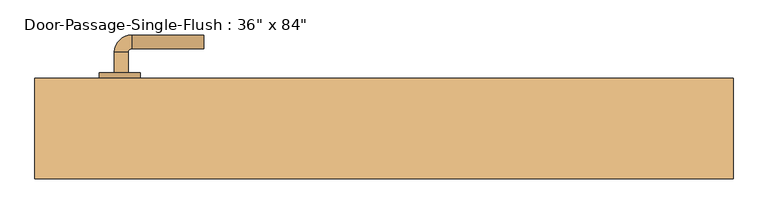
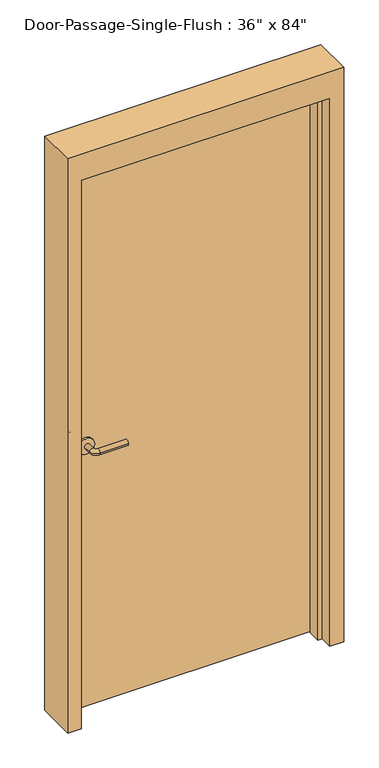
"""IFC4 building model written with IfcOpenShell, lengths in millimetres: door geometry."""

from ifc_helpers import new_model, si_unit, point, frame, frame_2d, origin, origin_with_axes, place, context, project, spatial, polyline, circle_curve, ellipse_curve, trimmed, segment, composite_curve, outline, extrude, faceted_brep, source, transform, mapped, element, save
from ifc_brep_helpers import plane_surface, cylinder_surface, revolved_surface, advanced_brep


def door_a46f4f49(model_context):
    return source(origin(), model_context, "Body", "SolidModel", [
        advanced_brep(
        [(-392.190625, 23.75, 1016.0), (-372.190625, 23.75, 1016.0), (-372.190625, -6.25, 1016.0), (-392.190625, -6.25, 1016.0), (-367.190625, -11.25, 1016.0), (-367.190625, -31.25, 1016.0), (-262.190625, -31.25, 1016.0), (-262.190625, -11.25, 1016.0)],
        [
            (0, 1, circle_curve(frame((-382.190625, 23.75, 1016.0), z_axis=(0.0, 1.0, 0.0), x_axis=(1.0, 0.0, 0.0)), 10.0)),
            (1, 0, circle_curve(frame((-382.190625, 23.75, 1016.0), z_axis=(0.0, 1.0, 0.0), x_axis=(1.0, 0.0, 0.0)), 10.0)),
            (1, 2),
            (2, 3, circle_curve(frame((-382.190625, -6.25, 1016.0), z_axis=(0.0, 1.0, 0.0), x_axis=(1.0, 0.0, 0.0)), 10.0)),
            (3, 0),
            (3, 2, circle_curve(frame((-382.190625, -6.25, 1016.0), z_axis=(0.0, 1.0, 0.0), x_axis=(1.0, 0.0, 0.0)), 10.0)),
            (4, 5, circle_curve(frame((-367.190625, -21.25, 1016.0), z_axis=(-1.0, 0.0, 0.0), x_axis=(0.0, 1.0, 0.0)), 10.0)),
            (5, 3, circle_curve(frame((-367.190625, -6.25, 1016.0), z_axis=(0.0, 0.0, -1.0), x_axis=(-1.0, 0.0, 0.0)), 25.0)),
            (2, 4, circle_curve(frame((-367.190625, -6.25, 1016.0), z_axis=(0.0, 0.0, 1.0), x_axis=(-1.0, 0.0, 0.0)), 5.0)),
            (5, 4, circle_curve(frame((-367.190625, -21.25, 1016.0), z_axis=(-1.0, 0.0, 0.0), x_axis=(0.0, 1.0, 0.0)), 10.0)),
            (6, 7, circle_curve(frame((-262.190625, -21.25, 1016.0), z_axis=(1.0, 0.0, 0.0), x_axis=(0.0, 1.0, 0.0)), 10.0)),
            (7, 6, circle_curve(frame((-262.190625, -21.25, 1016.0), z_axis=(1.0, 0.0, 0.0), x_axis=(0.0, 1.0, 0.0)), 10.0)),
            (4, 7),
            (6, 5),
        ],
        [
            plane_surface(frame((-382.190625, 23.75, 1016.0), z_axis=(0.0, 1.0, 0.0), x_axis=(0.0, 0.0, 1.0))),
            cylinder_surface(frame((-382.190625, 23.75, 1016.0), z_axis=(0.0, 1.0, 0.0), x_axis=(1.0, 0.0, 0.0)), 10.0),
            revolved_surface(trimmed(ellipse_curve(frame((-382.190625, -6.25, 1016.0), z_axis=(0.0, -1.0, 0.0), x_axis=(1.0, 0.0, 0.0)), 10.0, 10.0), [point((-392.190625, -6.25, 1016.0))], [point((-372.190625, -6.25, 1016.0))], True, "CARTESIAN"), (-367.190625, -6.25, 1016.0), (0.0, 0.0, -1.0)),
            revolved_surface(trimmed(ellipse_curve(frame((-382.190625, -6.25, 1016.0), z_axis=(0.0, -1.0, 0.0), x_axis=(1.0, 0.0, 0.0)), 10.0, 10.0), [point((-372.190625, -6.25, 1016.0))], [point((-392.190625, -6.25, 1016.0))], True, "CARTESIAN"), (-367.190625, -6.25, 1016.0), (0.0, 0.0, -1.0)),
            plane_surface(frame((-262.190625, -21.25, 1016.0), z_axis=(1.0, 0.0, 0.0), x_axis=(0.0, 0.0, 1.0))),
            cylinder_surface(frame((-367.190625, -21.25, 1016.0), z_axis=(-1.0, 0.0, 0.0), x_axis=(0.0, 1.0, 0.0)), 10.0),
        ],
        [
            (0, [[1, 2]]),
            (1, [[3, 4, 5, -2]]),
            (1, [[-5, 6, -3, -1]]),
            (2, [[7, 8, -4, 9]]),
            (3, [[10, -9, -6, -8]]),
            (4, [[11, 12]]),
            (5, [[13, -11, 14, -7]]),
            (5, [[-14, -12, -13, -10]]),
        ],
    ),
        extrude(outline(composite_curve([segment(trimmed(circle_curve(frame_2d((1016.0, -384.690625)), 30.0), [point((1016.0, -414.690625))], [point((1016.0, -354.690625))], False, "CARTESIAN"), True, "CONTINUOUS"), segment(trimmed(circle_curve(frame_2d((1016.0, -384.690625)), 30.0), [point((1016.0, -354.690625))], [point((1016.0, -414.690625))], False, "CARTESIAN"), True, "CONTINUOUS")], self_intersect=False)), frame((0.0, 23.75, 0.0), z_axis=(0.0, 1.0, 0.0), x_axis=(0.0, 0.0, 1.0)), (0.0, 0.0, 1.0), 8.0),
        advanced_brep(
        [(-392.190625, 84.2, 1016.0), (-372.190625, 84.2, 1016.0), (-392.190625, 114.2, 1016.0), (-372.190625, 114.2, 1016.0), (-367.190625, 119.2, 1016.0), (-367.190625, 139.2, 1016.0), (-262.190625, 139.2, 1016.0), (-262.190625, 119.2, 1016.0)],
        [
            (0, 1, circle_curve(frame((-382.190625, 84.2, 1016.0), z_axis=(0.0, -1.0, 0.0), x_axis=(1.0, 0.0, 0.0)), 10.0)),
            (1, 0, circle_curve(frame((-382.190625, 84.2, 1016.0), z_axis=(0.0, -1.0, 0.0), x_axis=(1.0, 0.0, 0.0)), 10.0)),
            (0, 2),
            (2, 3, circle_curve(frame((-382.190625, 114.2, 1016.0), z_axis=(0.0, -1.0, 0.0), x_axis=(1.0, 0.0, 0.0)), 10.0)),
            (3, 1),
            (3, 2, circle_curve(frame((-382.190625, 114.2, 1016.0), z_axis=(0.0, -1.0, 0.0), x_axis=(1.0, 0.0, 0.0)), 10.0)),
            (4, 3, circle_curve(frame((-367.190625, 114.2, 1016.0), z_axis=(0.0, 0.0, 1.0), x_axis=(-1.0, 0.0, 0.0)), 5.0)),
            (2, 5, circle_curve(frame((-367.190625, 114.2, 1016.0), z_axis=(0.0, 0.0, -1.0), x_axis=(-1.0, 0.0, 0.0)), 25.0)),
            (5, 4, circle_curve(frame((-367.190625, 129.2, 1016.0), z_axis=(-1.0, 0.0, 0.0), x_axis=(0.0, -1.0, 0.0)), 10.0)),
            (4, 5, circle_curve(frame((-367.190625, 129.2, 1016.0), z_axis=(-1.0, 0.0, 0.0), x_axis=(0.0, -1.0, 0.0)), 10.0)),
            (6, 7, circle_curve(frame((-262.190625, 129.2, 1016.0), z_axis=(1.0, 0.0, 0.0), x_axis=(0.0, -1.0, 0.0)), 10.0)),
            (7, 6, circle_curve(frame((-262.190625, 129.2, 1016.0), z_axis=(1.0, 0.0, 0.0), x_axis=(0.0, -1.0, 0.0)), 10.0)),
            (5, 6),
            (7, 4),
        ],
        [
            plane_surface(frame((-382.190625, 84.2, 1016.0), z_axis=(0.0, -1.0, 0.0), x_axis=(0.0, 0.0, 1.0))),
            cylinder_surface(frame((-382.190625, 84.2, 1016.0), z_axis=(0.0, -1.0, 0.0), x_axis=(1.0, 0.0, 0.0)), 10.0),
            revolved_surface(trimmed(ellipse_curve(frame((-382.190625, 114.2, 1016.0), z_axis=(0.0, -1.0, 0.0), x_axis=(1.0, 0.0, 0.0)), 10.0, 10.0), [point((-392.190625, 114.2, 1016.0))], [point((-372.190625, 114.2, 1016.0))], True, "CARTESIAN"), (-367.190625, 114.2, 1016.0), (0.0, 0.0, -1.0)),
            revolved_surface(trimmed(ellipse_curve(frame((-382.190625, 114.2, 1016.0), z_axis=(0.0, -1.0, 0.0), x_axis=(1.0, 0.0, 0.0)), 10.0, 10.0), [point((-372.190625, 114.2, 1016.0))], [point((-392.190625, 114.2, 1016.0))], True, "CARTESIAN"), (-367.190625, 114.2, 1016.0), (0.0, 0.0, -1.0)),
            plane_surface(frame((-262.190625, 129.2, 1016.0), z_axis=(1.0, 0.0, 0.0), x_axis=(0.0, 0.0, 1.0))),
            cylinder_surface(frame((-367.190625, 129.2, 1016.0), z_axis=(-1.0, 0.0, 0.0), x_axis=(0.0, -1.0, 0.0)), 10.0),
        ],
        [
            (0, [[1, 2]]),
            (1, [[-1, 3, 4, 5]]),
            (1, [[-2, -5, 6, -3]]),
            (2, [[7, -4, 8, 9]]),
            (3, [[-8, -6, -7, 10]]),
            (4, [[11, 12]]),
            (5, [[-9, 13, -12, 14]]),
            (5, [[-10, -14, -11, -13]]),
        ],
    ),
        extrude(outline(composite_curve([segment(trimmed(circle_curve(frame_2d((1016.0, -384.690625)), 30.0), [point((1016.0, -414.690625))], [point((1016.0, -354.690625))], False, "CARTESIAN"), True, "CONTINUOUS"), segment(trimmed(circle_curve(frame_2d((1016.0, -384.690625)), 30.0), [point((1016.0, -354.690625))], [point((1016.0, -414.690625))], False, "CARTESIAN"), True, "CONTINUOUS")], self_intersect=False)), frame((0.0, 76.2, 0.0), z_axis=(0.0, 1.0, 0.0), x_axis=(0.0, 0.0, 1.0)), (0.0, 0.0, 1.0), 8.0),
        faceted_brep([(457.2, 26.9875, 0.0), (457.2, 76.2, 0.0), (508.0, 76.2, 0.0), (508.0, -69.85, 0.0), (457.2, -69.85, 0.0), (457.2, -20.6375, 0.0), (441.325, -20.6375, 0.0), (441.325, 26.9875, 0.0), (457.2, 26.9875, 2133.6), (457.2, 76.2, 2133.6), (-457.2, 76.2, 2133.6), (-457.2, 76.2, 0.0), (-508.0, 76.2, 0.0), (-508.0, 76.2, 2235.2), (508.0, 76.2, 2235.2), (508.0, -69.85, 2235.2), (-508.0, -69.85, 2235.2), (-508.0, -69.85, 0.0), (-457.2, -69.85, 0.0), (-457.2, -69.85, 2133.6), (457.2, -69.85, 2133.6), (457.2, -20.6375, 2133.6), (-457.2, -20.6375, 2133.6), (-457.2, -20.6375, 0.0), (-441.325, -20.6375, 0.0), (-441.325, -20.6375, 2117.725), (441.325, -20.6375, 2117.725), (441.325, 26.9875, 2117.725), (-441.325, 26.9875, 2117.725), (-441.325, 26.9875, 0.0), (-457.2, 26.9875, 0.0), (-457.2, 26.9875, 2133.6)], [[[0, 1, 2, 3, 4, 5, 6, 7]], [[1, 0, 8, 9]], [[2, 1, 9, 10, 11, 12, 13, 14]], [[3, 2, 14, 15]], [[4, 3, 15, 16, 17, 18, 19, 20]], [[5, 4, 20, 21]], [[6, 5, 21, 22, 23, 24, 25, 26]], [[7, 6, 26, 27]], [[0, 7, 27, 28, 29, 30, 31, 8]], [[9, 8, 31, 10]], [[20, 19, 22, 21]], [[26, 25, 28, 27]], [[12, 11, 30, 29, 24, 23, 18, 17]], [[11, 10, 31, 30]], [[13, 12, 17, 16]], [[19, 18, 23, 22]], [[25, 24, 29, 28]], [[15, 14, 13, 16]]]),
        extrude(outline(polyline([(457.2, 31.75), (-457.2, 31.75), (-457.2, 76.2), (457.2, 76.2), (457.2, 31.75)])), origin_with_axes(), (0.0, 0.0, 1.0), 2133.6),
    ])


if __name__ == "__main__":
    model = new_model("IFC4")
    model_context = context("Model", 3, world=origin())
    ifc_project = project(units=[si_unit("LENGTHUNIT", "METRE", prefix="MILLI")], contexts=[model_context])
    site = spatial("IfcSite", under=ifc_project)
    building = spatial("IfcBuilding", under=site)
    placement = place(None, origin())
    door_shape = door_a46f4f49(model_context)
    element("IfcDoor", 1, ObjectType="Door-Passage-Single-Flush : 36\" x 84\"", at=placement, inside=building, context=model_context, shape_type="MappedRepresentation", body=[
        mapped(door_shape, transform((0.0, 0.0, 0.0), x_axis=(1.0, 0.0, 0.0), y_axis=(0.0, 1.0, 0.0), z_axis=(0.0, 0.0, 1.0))),
    ])
    save(model, "model.ifc")

# Revit data of these elements
# Type "Door-Passage-Single-Flush : 36\" x 84\""
#   Type Mark = "35"
#   Assembly Code = "B2030200"
#   Analytic Construction = "Wooden"
#   Thickness = 0' - 1 3/4"
#   Thermal Resistance (R) = 2.5876 (h·ft²·°F)/BTU
#   Swing Angle [instance default] = 90.00°
#   Strike Height = 3' - 4"
#   Rough Width [instance default] = 3' - 4"
#   Rough Height [instance default] = 7' - 4"
#   MF Opening Height [instance default] = 0' - 4"
#   MF Opening Width [instance default] = 0' - 4"
#   Inset Calculate [instance default] = 0' - 4"
#   Masonry Inset [instance default] = 0' - 1"
#   Height = 7' - 0"
#   Width = 3' - 0"
#   Heat Transfer Coefficient (U) = 0.3865 BTU/(h·ft²·°F)
#   Masonry Frame Depth = 0' - 5 3/4"
#   Masonry Frame [instance default] = yes
#   Function = 1
#   Dry Wall Frame [instance default] = no
#   Panel Material = Wood - Birch
#   Frame Material = Metal - Paint Finish - Grey
#   Door Handle Material = Aluminum
#   Visual Light Transmittance = 0
#   Solar Heat Gain Coefficient = 0
#   Wall Closure = (empty or 0)
# Element 1 (IfcDoor, "Door-Passage-Single-Flush : 36\" x 84\"")
#   Inset Calculate = 0' - 3"
#   Masonry Inset = 0' - 0"
#   Materials on its faces: "Aluminum", "Metal - Paint Finish - Grey", "Wood - Birch"
# Materials
#   "Wood - Birch": class "Wood", colour RGB 166 116 52, transparency 0, Cost = 0
#   "Metal - Paint Finish - Grey": class "Paint", colour RGB 104 104 104, transparency 0, Cost = 0
#   "Aluminum": class "Metal", colour RGB 247 247 247, transparency 0, Description = "Aluminum 6061", Cost = 0
